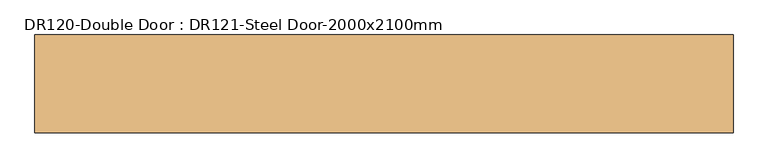
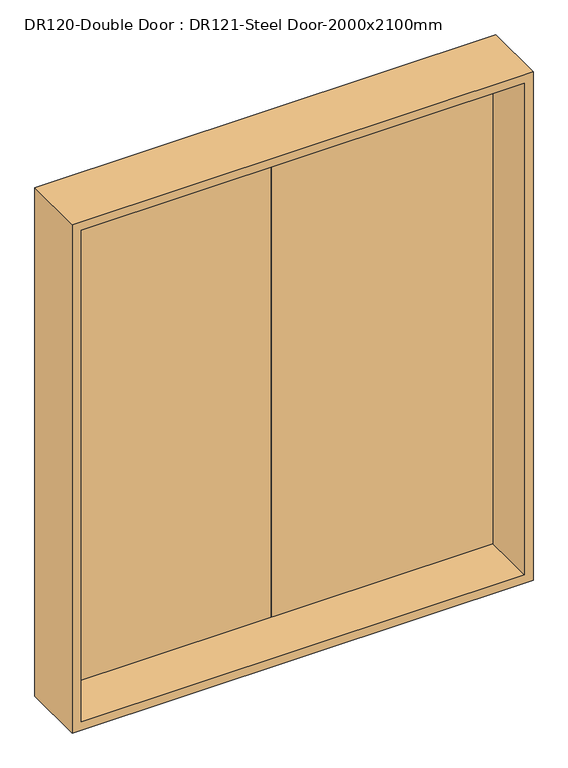
"""IFC4 building model written with IfcOpenShell, lengths in millimetres: door geometry, DR120-Double Door : DR121-Steel Door-2000x2100mm."""

from ifc_helpers import new_model, si_unit, frame, origin, place, context, project, spatial, polyline, outline, extrude, faceted_brep, source, transform, mapped, element, save


def dr120_double_door_dr121_steel_door_2000x2100mm_b0f5a95a(model_context):
    return source(origin(), model_context, "Body", "SolidModel", [
        extrude(outline(polyline([(880.0, 86.0), (0.0, 86.0), (0.0, 126.0), (880.0, 126.0), (880.0, 86.0)])), frame((0.0, 0.0, 20.0), z_axis=(0.0, 0.0, 1.0), x_axis=(1.0, 0.0, 0.0)), (0.0, 0.0, 1.0), 2060.0),
        extrude(outline(polyline([(0.0, 86.0), (-880.0, 86.0), (-880.0, 126.0), (0.0, 126.0), (0.0, 86.0)])), frame((0.0, 0.0, 20.0), z_axis=(0.0, 0.0, 1.0), x_axis=(1.0, 0.0, 0.0)), (0.0, 0.0, 1.0), 2060.0),
        faceted_brep([(900.0, -126.0, 2100.0), (900.0, 126.0, 2100.0), (-900.0, 126.0, 2100.0), (-900.0, -126.0, 2100.0), (865.0, 86.0, 2065.0), (865.0, -126.0, 2065.0), (-865.0, -126.0, 2065.0), (-865.0, 86.0, 2065.0), (880.0, 126.0, 2080.0), (880.0, 86.0, 2080.0), (-880.0, 86.0, 2080.0), (-880.0, 126.0, 2080.0), (-900.0, 126.0, 0.0), (-900.0, -126.0, 0.0), (-865.0, -126.0, 35.0), (-865.0, 86.0, 35.0), (-880.0, 86.0, 20.0), (-880.0, 126.0, 20.0), (900.0, 126.0, 0.0), (880.0, 126.0, 20.0), (900.0, -126.0, 0.0), (865.0, -126.0, 35.0), (865.0, 86.0, 35.0), (880.0, 86.0, 20.0)], [[[0, 1, 2, 3]], [[4, 5, 6, 7]], [[8, 9, 10, 11]], [[3, 2, 12, 13]], [[7, 6, 14, 15]], [[11, 10, 16, 17]], [[18, 12, 2, 1], [8, 11, 17, 19]], [[13, 12, 18, 20]], [[0, 3, 13, 20], [21, 14, 6, 5]], [[15, 14, 21, 22]], [[23, 16, 10, 9], [4, 7, 15, 22]], [[17, 16, 23, 19]], [[20, 18, 1, 0]], [[22, 21, 5, 4]], [[19, 23, 9, 8]]]),
    ])


if __name__ == "__main__":
    model = new_model("IFC4")
    model_context = context("Model", 3, world=origin())
    ifc_project = project(units=[si_unit("LENGTHUNIT", "METRE", prefix="MILLI")], contexts=[model_context])
    site = spatial("IfcSite", under=ifc_project)
    building = spatial("IfcBuilding", under=site)
    placement = place(None, origin())
    dr120_double_door_dr121_steel_door_2000x2100mm_shape = dr120_double_door_dr121_steel_door_2000x2100mm_b0f5a95a(model_context)
    element("IfcDoor", 1, ObjectType="DR120-Double Door : DR121-Steel Door-2000x2100mm", at=placement, inside=building, context=model_context, shape_type="MappedRepresentation", body=[
        mapped(dr120_double_door_dr121_steel_door_2000x2100mm_shape, transform((0.0, 0.0, 0.0), x_axis=(1.0, 0.0, 0.0), y_axis=(0.0, 1.0, 0.0), z_axis=(0.0, 0.0, 1.0))),
    ])
    save(model, "model.ifc")

# Revit data of these elements
# Type "DR120-Double Door : DR121-Steel Door-2000x2100mm"
#   Type Mark = "SD"
#   프레임 = ""
#   철물 = ""
#   유리/마감 = ""
#   위치/개소 = ""
#   부호 = "1/SD"
#   문번호 = ""
#   문기호 = "SD"
#   Analytic Construction = "<None>"
#   Height = 2100 mm
#   Width = 1800 mm
#   Define Thermal Properties by = 1
#   문 틀 = A04AQ098-00003_Steel Door_non FP_double
#   문 = 문
#   Function = (empty or 0)
#   Assembly Code = ""
#   Wall Closure = (empty or 0)
# Element 1 (IfcDoor, "DR120-Double Door : DR121-Steel Door-2000x2100mm")
#   Materials on its faces: "A04AQ098-00003_Steel Door_non FP_double", "문"
# Materials
#   "A04AQ098-00003_Steel Door_non FP_double": class "금속", colour RGB 247 247 247, transparency 0, Description = "Steel Door", W00) Work Master Code = "A04AQ098-00003", W01) Work Master_Lv1 = "Finishing Work", W02) Work Master_Lv2 = "Door & Window Work", W03) Work Master_Spec.1 = "Steel Door w/ Steel Frame", W04) Work Master_Spec.2 = "Fire Protective Rating: N/A, Double Door", W05) Work Master_Spec.3 = "w/ Hardware & Accessories", Cost = 0
#   "문": class "다양한", colour RGB 247 247 247, transparency 0
